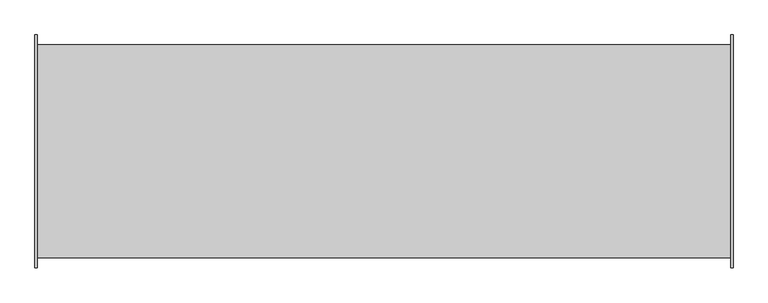
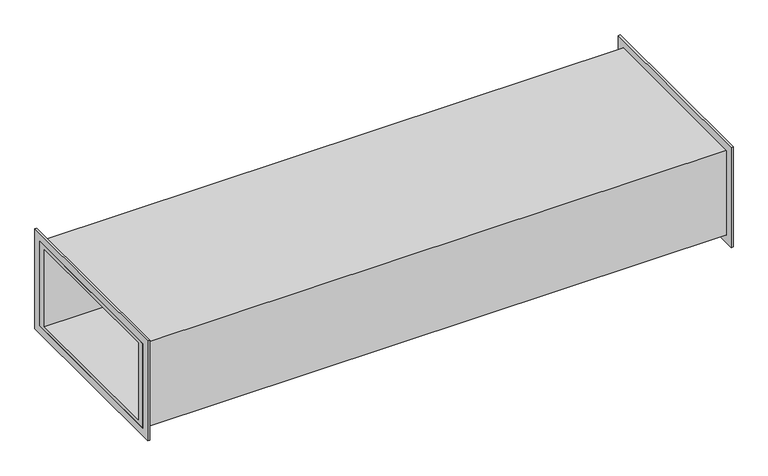
"""IFC4 building model written with IfcOpenShell, lengths in millimetres: proxy geometry, Бактерицидная секция BAW : Канальная бактерицидная секция BAW 40-20/9."""

from ifc_helpers import new_model, si_unit, frame, origin, place, context, project, spatial, polyline, outline, extrude, source, transform, mapped, element, save


def mechanical_equipment_f8aa3bbb(model_context):
    return source(origin(), model_context, "Body", "SweptSolid", [
        extrude(outline(polyline([(-240.0, 130.0), (240.0, 130.0), (240.0, -130.0), (-240.0, -130.0), (-240.0, 130.0)]), holes=[polyline([(-220.0, -110.0), (220.0, -110.0), (220.0, 110.0), (-220.0, 110.0), (-220.0, -110.0)])]), frame((715.0, 0.0, 0.0), z_axis=(1.0, 0.0, 0.0), x_axis=(0.0, 1.0, 0.0)), (0.0, 0.0, 1.0), 5.0),
        extrude(outline(polyline([(240.0, -130.0), (-240.0, -130.0), (-240.0, 130.0), (240.0, 130.0), (240.0, -130.0)]), holes=[polyline([(220.0, 110.0), (-220.0, 110.0), (-220.0, -110.0), (220.0, -110.0), (220.0, 110.0)])]), frame((-720.0, 0.0, 0.0), z_axis=(1.0, 0.0, 0.0), x_axis=(0.0, 1.0, 0.0)), (0.0, 0.0, 1.0), 5.0),
        extrude(outline(polyline([(220.0, 110.0), (220.0, -110.0), (-220.0, -110.0), (-220.0, 110.0), (220.0, 110.0)]), holes=[polyline([(200.0, 100.0), (-200.0, 100.0), (-200.0, -100.0), (200.0, -100.0), (200.0, 100.0)])]), frame((-720.0, 0.0, 0.0), z_axis=(1.0, 0.0, 0.0), x_axis=(0.0, 1.0, 0.0)), (0.0, 0.0, 1.0), 1440.0),
    ])


if __name__ == "__main__":
    model = new_model("IFC4")
    model_context = context("Model", 3, world=origin())
    ifc_project = project(units=[si_unit("LENGTHUNIT", "METRE", prefix="MILLI")], contexts=[model_context])
    site = spatial("IfcSite", under=ifc_project)
    building = spatial("IfcBuilding", under=site)
    placement = place(None, origin())
    mechanical_equipment_shape = mechanical_equipment_f8aa3bbb(model_context)
    element("IfcBuildingElementProxy", 1, Name="Бактерицидная секция BAW : Канальная бактерицидная секция BAW 40-20/9", ObjectType="Бактерицидная секция BAW : Канальная бактерицидная секция BAW 40-20/9", at=placement, inside=building, context=model_context, shape_type="MappedRepresentation", body=[
        mapped(mechanical_equipment_shape, transform((0.0, 0.0, 0.0), x_axis=(1.0, 0.0, 0.0), y_axis=(0.0, 1.0, 0.0), z_axis=(0.0, 0.0, 1.0))),
    ])
    save(model, "model.ifc")

# Revit data of these elements
# Type "Бактерицидная секция BAW : Канальная бактерицидная секция BAW 40-20/9"
#   ADSK_Система_Имя [instance default] = ""
#   ADSK_Наименование краткое = "BAW 40-20/9"
#   ADSK_Наименование [instance default] = "Канальная бактерицидная секция BAW 40-20/9"
#   ADSK_Масса_Текст = "30.2"
#   ADSK_Марка = "BAW 40-20/9"
#   ADSK_Код изделия = "Канальная бактерицидная секция BAW 40-20/9"
#   ADSK_Завод-изготовитель = "WAER"
#   ADSK_Единица измерения = "шт."
#   ADSK_URL страницы изделия = "https://waer-air.com/baktericidnye-sekcii-baw/"
#   ADSK_URL документации изделия = ""
#   ADSK_Ток = 3.06 A
#   ADSK_Расход воздуха = 300 m³/h
#   ADSK_Размер_Ширина_Д = 440 mm
#   ADSK_Размер_Ширина_А = 400 mm
#   ADSK_Размер_Высота_Г = 220 mm
#   ADSK_Размер_Высота_Б = 200 mm
#   ADSK_Потеря давления воздуха = 0.0 Pa
#   ADSK_Полная мощность = 673.2 VA
#   ADSK_Номинальная мощность = 675 W
#   ADSK_Напряжение = 220 V
#   ADSK_Масса = 30.2
#   ADSK_Количество ламп = 9
#   ADSK_Количество [instance default] = 1
#   ADSK_Бактерицидный поток = 238.5
#   ADSK_Количество фаз = 1
#   ADSK_Классификация нагрузок = ОВК
#   Default Elevation = 0
#   URL = ""
#   Cost = 0
